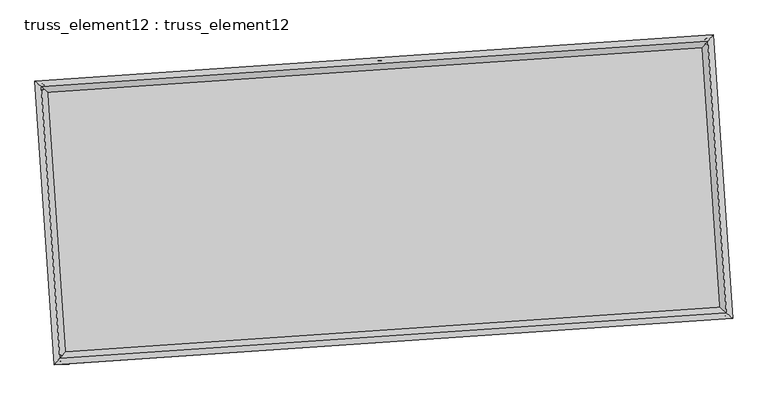
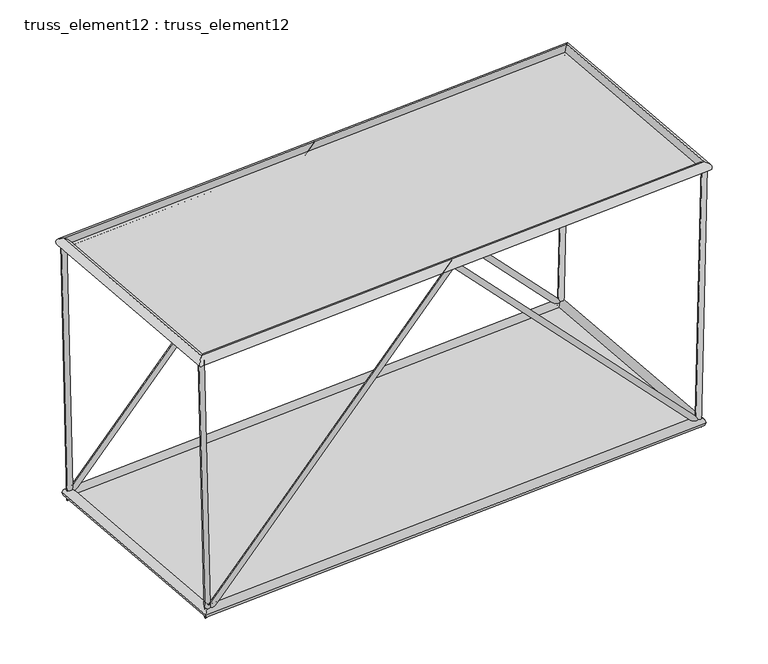
"""IFC4 building model written with IfcOpenShell, lengths in millimetres: plate geometry, truss_element12 : truss_element12."""

from ifc_helpers import new_model, si_unit, frame, origin, origin_with_axes, place, context, project, spatial, polyline, circle_curve, ellipse_curve, outline, extrude, source, transform, mapped, element, save
from ifc_brep_helpers import plane_surface, cylinder_surface, advanced_brep


def truss_element12_truss_element12_fedef946(model_context):
    return source(origin(), model_context, "Body", "SolidModel", [
        advanced_brep(
        [(-3782.029021, 2268.2402197, 4999.7937205), (-3881.1049687, 2254.8808593, 4997.4519118), (-3667.7673536, 2276.0312884, 121.2284017), (-3761.2195292, 2263.0553917, -121.2284017), (1063.6545258, 2598.6489605, 5070.7379406), (1064.1036954, 2592.0758396, 4926.5107213), (5795.2031248, 2921.2752732, 121.229281), (5889.5578522, 2921.1052153, -121.229281), (5909.3390115, 2929.0577654, 4999.7954616), (6009.3114208, 2929.2707559, 4997.4562298)],
        [
            (0, 1, circle_curve(frame((-3831.5669949, 2261.5605395, 4998.6228161), z_axis=(-0.02341471068854239, -0.0015965601142035673, 0.9997245632268789), x_axis=(-0.1335941952691201, 0.9910349136664861, -0.0015462485106522157)), 50.0)),
            (1, 0, circle_curve(frame((-3831.5669949, 2261.5605395, 4998.6228161), z_axis=(-0.02341471068854239, -0.0015965601142035673, 0.9997245632268789), x_axis=(-0.1335941952691201, 0.9910349136664861, -0.0015462485106522157)), 50.0)),
            (0, 2),
            (2, 3, ellipse_curve(frame((-3714.4934414, 2269.54334, 0.0), z_axis=(-0.9300661480063914, -0.06341767512013644, 0.36187727037617307), x_axis=(0.3610389440712066, 0.024617873158703073, 0.9322257458282786)), 130.3250571, 50.0)),
            (3, 1),
            (3, 2, ellipse_curve(frame((-3714.4934414, 2269.54334, 0.0), z_axis=(-0.9300661480063914, -0.06341767512013644, 0.36187727037617307), x_axis=(0.3610389440712066, 0.024617873158703073, 0.9322257458282786)), 130.3250571, 50.0)),
            (2, 4),
            (4, 5, ellipse_curve(frame((1063.8791106, 2595.3624001, 4998.6243309), z_axis=(-0.9976833960522568, -0.06802823822716046, -6.7338070324165216e-06), x_axis=(6.718207468311702e-06, 4.5808902877525703e-07, -0.9999999999773279)), 72.2706352, 50.0)),
            (5, 3),
            (5, 4, ellipse_curve(frame((1063.8791106, 2595.3624001, 4998.6243309), z_axis=(-0.9976833960522568, -0.06802823822716046, -6.7338070324165216e-06), x_axis=(6.718207468311702e-06, 4.5808902877525703e-07, -0.9999999999773279)), 72.2706352, 50.0)),
            (4, 6),
            (6, 7, ellipse_curve(frame((5842.3804885, 2921.1902443, 0.0), z_axis=(-0.9300590534640555, -0.06341719137026322, -0.3618955884067292), x_axis=(-0.36105721966614135, -0.02461911930204943, 0.9322186348125355)), 130.3269965, 50.0)),
            (7, 5),
            (7, 6, ellipse_curve(frame((5842.3804885, 2921.1902443, 0.0), z_axis=(-0.9300590534640555, -0.06341719137026322, -0.3618955884067292), x_axis=(-0.36105721966614135, -0.02461911930204943, 0.9322186348125355)), 130.3269965, 50.0)),
            (8, 9, circle_curve(frame((5959.3252161, 2929.1642607, 4998.6258457), z_axis=(0.023388945526827118, 0.0015948032857688488, 0.9997251691488132), x_axis=(-0.002166625472093405, 0.9999964600479803, -0.0015445470442767841)), 50.0)),
            (9, 8, circle_curve(frame((5959.3252161, 2929.1642607, 4998.6258457), z_axis=(0.023388945526827118, 0.0015948032857688488, 0.9997251691488132), x_axis=(-0.002166625472093405, 0.9999964600479803, -0.0015445470442767841)), 50.0)),
            (6, 8),
            (9, 7),
        ],
        [
            plane_surface(frame((-3831.5669949, 2311.5604757, 4998.702666), z_axis=(-0.023414710688541198, -0.0015965601141989434, 0.999724563226879), x_axis=(0.9997258380793066, -3.739324497509243e-05, 0.02341468083005437))),
            cylinder_surface(frame((-3831.5669949, 2261.5605395, 4998.6228161), z_axis=(-0.02341471068854239, -0.0015965601142035673, 0.9997245632268789), x_axis=(-0.1335941952691201, 0.9910349136664861, -0.0015462485106522157)), 50.0),
            cylinder_surface(frame((-3714.4934414, 2269.54334, 0.0), z_axis=(-0.6902363467958819, -0.047064592654016545, -0.7220517361520478), x_axis=(-0.020418619460760453, 0.9987519259602177, -0.04558146959096984)), 50.0),
            cylinder_surface(frame((1063.8791106, 2595.3624001, 4998.6243309), z_axis=(-0.6902460485200185, -0.04706525417770545, 0.722042418665059), x_axis=(-0.11534162865299183, 0.9922794867995385, -0.04558211026839251)), 50.0),
            plane_surface(frame((5959.3252161, 2879.1643243, 4998.7056077), z_axis=(0.023388945526829154, 0.0015948032857737223, 0.9997251691488129), x_axis=(0.999726441196362, -3.731097392289939e-05, -0.023388915766837215))),
            cylinder_surface(frame((5842.3804885, 2921.1902443, 0.0), z_axis=(-0.023388945526827118, -0.0015948032857688488, -0.9997251691488132), x_axis=(-0.002166625472093405, 0.9999964600479803, -0.0015445470442767841)), 50.0),
        ],
        [
            (0, [[1, 2]]),
            (1, [[-1, 3, 4, 5]]),
            (1, [[-2, -5, 6, -3]]),
            (2, [[-4, 7, 8, 9]]),
            (2, [[-6, -9, 10, -7]]),
            (3, [[-8, 11, 12, 13]]),
            (3, [[-10, -13, 14, -11]]),
            (4, [[15, 16]]),
            (5, [[-12, 17, -16, 18]]),
            (5, [[-14, -18, -15, -17]]),
        ],
    ),
        advanced_brep(
        [(-3509.9160681, -1722.4933646, 4999.7937205), (-3608.9920158, -1735.852725, 4997.4519118), (-3395.6544007, -1714.7022959, 121.2284017), (-3489.1065763, -1727.6781926, -121.2284017), (1335.7674788, -1392.0846238, 5070.7379406), (1336.2166483, -1398.6577447, 4926.5107213), (6067.3160777, -1069.4583111, 121.229281), (6161.6708052, -1069.628369, -121.229281), (6181.4519644, -1061.6758189, 4999.7954616), (6281.4243737, -1061.4628284, 4997.4562298)],
        [
            (0, 1, circle_curve(frame((-3559.4540419, -1729.1730448, 4998.6228161), z_axis=(-0.023414710688542402, -0.0015965601142035601, 0.999724563226879), x_axis=(-0.13359419526911945, 0.9910349136664863, -0.001546248510652208)), 50.0)),
            (1, 0, circle_curve(frame((-3559.4540419, -1729.1730448, 4998.6228161), z_axis=(-0.023414710688542402, -0.0015965601142035601, 0.999724563226879), x_axis=(-0.13359419526911945, 0.9910349136664863, -0.001546248510652208)), 50.0)),
            (0, 2),
            (2, 3, ellipse_curve(frame((-3442.3804885, -1721.1902443, 0.0), z_axis=(-0.9300661480063912, -0.06341767512013613, 0.36187727037617334), x_axis=(0.3610389440712068, 0.024617873158702973, 0.9322257458282784)), 130.3250571, 50.0)),
            (3, 1),
            (3, 2, ellipse_curve(frame((-3442.3804885, -1721.1902443, 0.0), z_axis=(-0.9300661480063912, -0.06341767512013613, 0.36187727037617334), x_axis=(0.3610389440712068, 0.024617873158702973, 0.9322257458282784)), 130.3250571, 50.0)),
            (2, 4),
            (4, 5, ellipse_curve(frame((1335.9920636, -1395.3711842, 4998.6243309), z_axis=(-0.997683396052257, -0.0680282382271604, -6.733807032095577e-06), x_axis=(6.718207468465462e-06, 4.5808902903472784e-07, -0.9999999999773279)), 72.2706352, 50.0)),
            (5, 3),
            (5, 4, ellipse_curve(frame((1335.9920636, -1395.3711842, 4998.6243309), z_axis=(-0.997683396052257, -0.0680282382271604, -6.733807032095577e-06), x_axis=(6.718207468465462e-06, 4.5808902903472784e-07, -0.9999999999773279)), 72.2706352, 50.0)),
            (4, 6),
            (6, 7, ellipse_curve(frame((6114.4934414, -1069.54334, 0.0), z_axis=(-0.9300590534640557, -0.06341719137026328, -0.3618955884067287), x_axis=(-0.36105721966614074, -0.02461911930204951, 0.9322186348125356)), 130.3269965, 50.0)),
            (7, 5),
            (7, 6, ellipse_curve(frame((6114.4934414, -1069.54334, 0.0), z_axis=(-0.9300590534640557, -0.06341719137026328, -0.3618955884067287), x_axis=(-0.36105721966614074, -0.02461911930204951, 0.9322186348125356)), 130.3269965, 50.0)),
            (8, 9, circle_curve(frame((6231.4381691, -1061.5693236, 4998.6258457), z_axis=(0.023388945526827663, 0.0015948032857688026, 0.999725169148813), x_axis=(-0.002166625472094084, 0.9999964600479802, -0.001544547044276721)), 50.0)),
            (9, 8, circle_curve(frame((6231.4381691, -1061.5693236, 4998.6258457), z_axis=(0.023388945526827663, 0.0015948032857688026, 0.999725169148813), x_axis=(-0.002166625472094084, 0.9999964600479802, -0.001544547044276721)), 50.0)),
            (6, 8),
            (9, 7),
        ],
        [
            plane_surface(frame((-3559.4540419, -1679.1731086, 4998.702666), z_axis=(-0.023414710688541198, -0.0015965601141989477, 0.999724563226879), x_axis=(0.9997258380793066, -3.739324497509243e-05, 0.02341468083005437))),
            cylinder_surface(frame((-3559.4540419, -1729.1730448, 4998.6228161), z_axis=(-0.023414710688542402, -0.0015965601142035601, 0.999724563226879), x_axis=(-0.13359419526911945, 0.9910349136664863, -0.001546248510652208)), 50.0),
            cylinder_surface(frame((-3442.3804885, -1721.1902443, 0.0), z_axis=(-0.6902363467958823, -0.047064592654016364, -0.7220517361520478), x_axis=(-0.020418619460760457, 0.9987519259602178, -0.04558146959096958)), 50.0),
            cylinder_surface(frame((1335.9920636, -1395.3711842, 4998.6243309), z_axis=(-0.6902460485200181, -0.04706525417770555, 0.7220424186650592), x_axis=(-0.11534162865299175, 0.9922794867995385, -0.04558211026839221)), 50.0),
            plane_surface(frame((6231.4381691, -1111.56926, 4998.7056077), z_axis=(0.02338894552682561, 0.0015948032857737312, 0.9997251691488132), x_axis=(0.9997264411963621, -3.731097392245531e-05, -0.023388915766833666))),
            cylinder_surface(frame((6114.4934414, -1069.54334, 0.0), z_axis=(-0.023388945526827663, -0.0015948032857688026, -0.999725169148813), x_axis=(-0.002166625472094084, 0.9999964600479802, -0.001544547044276721)), 50.0),
        ],
        [
            (0, [[1, 2]]),
            (1, [[-1, 3, 4, 5]]),
            (1, [[-2, -5, 6, -3]]),
            (2, [[-4, 7, 8, 9]]),
            (2, [[-6, -9, 10, -7]]),
            (3, [[-8, 11, 12, 13]]),
            (3, [[-10, -13, 14, -11]]),
            (4, [[15, 16]]),
            (5, [[-12, 17, -16, 18]]),
            (5, [[-14, -18, -15, -17]]),
        ],
    ),
        advanced_brep(
        [(-3559.4532557, -1729.1721734, 4908.6228161), (-3559.4548282, -1729.1739162, 5088.6228161), (-3831.5678921, 2261.5612961, 5088.6228161), (-3831.5660976, 2261.5597829, 4908.6228161), (5959.3259469, 2929.1651283, 5088.6258457), (5959.3244853, 2929.1633931, 4908.6258457), (6231.4390108, -1061.570084, 5088.6258457), (6231.4373273, -1061.5685632, 4908.6258457)],
        [
            (0, 1, ellipse_curve(frame((-3559.4540419, -1729.1730448, 4998.6228161), z_axis=(-0.7535719234054217, 0.657365466278086, -2.182941780963091e-07), x_axis=(-0.65736546627805, -0.7535719234054532, -2.1829417809634472e-07)), 127.2792206, 90.0)),
            (1, 2),
            (2, 3, ellipse_curve(frame((-3831.5669949, 2261.5605395, 4998.6228161), z_axis=(-0.65736546627805, -0.7535719234054532, -2.1829417809637778e-07), x_axis=(0.7535719234054218, -0.6573654662780859, 2.1829417809634224e-07)), 127.2792206, 90.0)),
            (3, 0),
            (1, 0, ellipse_curve(frame((-3559.4540419, -1729.1730448, 4998.6228161), z_axis=(-0.7535719234054217, 0.657365466278086, -2.182941780963091e-07), x_axis=(-0.65736546627805, -0.7535719234054532, -2.1829417809634472e-07)), 127.2792206, 90.0)),
            (3, 2, ellipse_curve(frame((-3831.5669949, 2261.5605395, 4998.6228161), z_axis=(-0.65736546627805, -0.7535719234054532, -2.1829417809637778e-07), x_axis=(0.7535719234054218, -0.6573654662780859, 2.1829417809634224e-07)), 127.2792206, 90.0)),
            (2, 4),
            (4, 5, ellipse_curve(frame((5959.3252161, 2929.1642607, 4998.6258457), z_axis=(-0.7535719234054216, 0.6573654662780861, -2.1829417809637545e-07), x_axis=(-0.6573654662780505, -0.7535719234054526, -2.182941780963446e-07)), 127.2792206, 90.0)),
            (5, 3),
            (5, 4, ellipse_curve(frame((5959.3252161, 2929.1642607, 4998.6258457), z_axis=(-0.7535719234054216, 0.6573654662780861, -2.1829417809637545e-07), x_axis=(-0.6573654662780505, -0.7535719234054526, -2.182941780963446e-07)), 127.2792206, 90.0)),
            (4, 6),
            (6, 7, ellipse_curve(frame((6231.4381691, -1061.5693236, 4998.6258457), z_axis=(0.6573654662780504, 0.7535719234054529, 2.1829417809631145e-07), x_axis=(-0.7535719234054216, 0.6573654662780863, -2.1829417809634234e-07)), 127.2792206, 90.0)),
            (7, 5),
            (7, 6, ellipse_curve(frame((6231.4381691, -1061.5693236, 4998.6258457), z_axis=(0.6573654662780504, 0.7535719234054529, 2.1829417809631145e-07), x_axis=(-0.7535719234054216, 0.6573654662780863, -2.1829417809634234e-07)), 127.2792206, 90.0)),
            (6, 1),
            (0, 7),
        ],
        [
            cylinder_surface(frame((-3559.4540419, -1729.1730448, 4998.6228161), z_axis=(0.06802823822869762, -0.997683396074877, 0.0), x_axis=(-0.9976833960310402, -0.06802823822570855, -9.37427355396142e-06)), 90.0),
            cylinder_surface(frame((-3831.5669949, 2261.5605395, 4998.6228161), z_axis=(-0.9976833960748294, -0.06802823822869407, -3.0871458725096017e-07), x_axis=(-0.06802823822310969, 0.9976833960340703, -9.06555896672317e-06)), 90.0),
            cylinder_surface(frame((5959.3252161, 2929.1642607, 4998.6258457), z_axis=(-0.06802823822869693, 0.9976833960748771, 0.0), x_axis=(0.9976833960366246, 0.06802823822608864, -8.75684437948492e-06)), 90.0),
            cylinder_surface(frame((6231.4381691, -1061.5693236, 4998.6258457), z_axis=(0.9976833960748294, 0.06802823822869393, 3.0871458725091337e-07), x_axis=(0.06802823822869393, -0.9976833960336895, -9.065558966723174e-06)), 90.0),
        ],
        [
            (0, [[1, 2, 3, 4]]),
            (0, [[5, -4, 6, -2]]),
            (1, [[-3, 7, 8, 9]]),
            (1, [[-6, -9, 10, -7]]),
            (2, [[-8, 11, 12, 13]]),
            (2, [[-10, -13, 14, -11]]),
            (3, [[-12, 15, -1, 16]]),
            (3, [[-14, -16, -5, -15]]),
        ],
    ),
        advanced_brep(
        [(-3358.7115243, -1625.2761972, 0.0), (-3526.0494527, -1817.1042913, 0.0), (-3810.4074885, 2353.2123043, 0.0), (-3618.5793943, 2185.8743758, 0.0), (5926.0494527, 3017.1042913, 0.0), (5758.7115243, 2825.2761972, 0.0), (6210.4074885, -1153.2123043, 0.0), (6018.5793943, -985.8743758, 0.0)],
        [
            (0, 1, ellipse_curve(frame((-3442.3804885, -1721.1902443, 0.0), z_axis=(-0.753571923405459, 0.6573654662780796, 0.0), x_axis=(-0.6573654662780796, -0.7535719234054591, 0.0)), 127.2792206, 90.0)),
            (1, 2),
            (2, 3, ellipse_curve(frame((-3714.4934414, 2269.54334, 0.0), z_axis=(-0.6573654662780795, -0.753571923405459, 0.0), x_axis=(0.7535719234054589, -0.6573654662780798, 0.0)), 127.2792206, 90.0)),
            (3, 0),
            (1, 0, ellipse_curve(frame((-3442.3804885, -1721.1902443, 0.0), z_axis=(-0.753571923405459, 0.6573654662780796, 0.0), x_axis=(-0.6573654662780796, -0.7535719234054591, 0.0)), 127.2792206, 90.0)),
            (3, 2, ellipse_curve(frame((-3714.4934414, 2269.54334, 0.0), z_axis=(-0.6573654662780795, -0.753571923405459, 0.0), x_axis=(0.7535719234054589, -0.6573654662780798, 0.0)), 127.2792206, 90.0)),
            (2, 4),
            (4, 5, ellipse_curve(frame((5842.3804885, 2921.1902443, 0.0), z_axis=(-0.753571923405459, 0.6573654662780796, 0.0), x_axis=(-0.6573654662780795, -0.753571923405459, 0.0)), 127.2792206, 90.0)),
            (5, 3),
            (5, 4, ellipse_curve(frame((5842.3804885, 2921.1902443, 0.0), z_axis=(-0.753571923405459, 0.6573654662780796, 0.0), x_axis=(-0.6573654662780795, -0.753571923405459, 0.0)), 127.2792206, 90.0)),
            (4, 6),
            (6, 7, ellipse_curve(frame((6114.4934414, -1069.54334, 0.0), z_axis=(0.6573654662780796, 0.7535719234054591, 0.0), x_axis=(-0.753571923405459, 0.6573654662780795, 0.0)), 127.2792206, 90.0)),
            (7, 5),
            (7, 6, ellipse_curve(frame((6114.4934414, -1069.54334, 0.0), z_axis=(0.6573654662780796, 0.7535719234054591, 0.0), x_axis=(-0.753571923405459, 0.6573654662780795, 0.0)), 127.2792206, 90.0)),
            (6, 1),
            (0, 7),
        ],
        [
            cylinder_surface(frame((-3442.3804885, -1721.1902443, 0.0), z_axis=(0.0680282382287029, -0.9976833960748764, 0.0), x_axis=(-0.9976833960748764, -0.0680282382287029, 0.0)), 90.0),
            cylinder_surface(frame((-3714.4934414, 2269.54334, 0.0), z_axis=(-0.9976833960748764, -0.06802823822870277, 0.0), x_axis=(-0.06802823822870277, 0.9976833960748764, 0.0)), 90.0),
            cylinder_surface(frame((5842.3804885, 2921.1902443, 0.0), z_axis=(-0.06802823822870296, 0.9976833960748764, 0.0), x_axis=(0.9976833960748764, 0.06802823822870296, 0.0)), 90.0),
            cylinder_surface(frame((6114.4934414, -1069.54334, 0.0), z_axis=(0.9976833960748764, 0.06802823822870276, 0.0), x_axis=(0.06802823822870276, -0.9976833960748764, 0.0)), 90.0),
        ],
        [
            (0, [[1, 2, 3, 4]]),
            (0, [[5, -4, 6, -2]]),
            (1, [[-3, 7, 8, 9]]),
            (1, [[-6, -9, 10, -7]]),
            (2, [[-8, 11, 12, 13]]),
            (2, [[-10, -13, 14, -11]]),
            (3, [[-12, 15, -1, 16]]),
            (3, [[-14, -16, -5, -15]]),
        ],
    ),
        extrude(outline(polyline([(-3442.3804885, -1721.1902443), (-3714.4934414, 2269.54334), (5842.3804885, 2921.1902443), (6114.4934414, -1069.54334), (-3442.3804885, -1721.1902443)])), origin_with_axes(), (0.0, 0.0, 1.0), 20.0),
        extrude(outline(polyline([(-2000.0, 4906.8132483), (2000.0000001, 4906.8132484), (2000.0000001, -4906.8132483), (-2000.0, -4906.8132484), (-2000.0, 4906.8132483)])), frame((1199.9355871, 599.9956079, 4998.6243309), z_axis=(-3.0799941782636826e-07, -2.100130948618238e-08, 0.9999999999999524), x_axis=(-0.06802823822870281, 0.9976833960748764, 0.0)), (0.0, 0.0, 1.0), 20.0),
    ])


if __name__ == "__main__":
    model = new_model("IFC4")
    model_context = context("Model", 3, world=origin())
    ifc_project = project(units=[si_unit("LENGTHUNIT", "METRE", prefix="MILLI")], contexts=[model_context])
    site = spatial("IfcSite", under=ifc_project)
    building = spatial("IfcBuilding", under=site)
    placement = place(None, origin())
    truss_element12_truss_element12_shape = truss_element12_truss_element12_fedef946(model_context)
    element("IfcPlate", 1, ObjectType="truss_element12 : truss_element12", at=placement, inside=building, context=model_context, shape_type="MappedRepresentation", body=[
        mapped(truss_element12_truss_element12_shape, transform((0.0, 0.0, 0.0), x_axis=(1.0, 0.0, 0.0), y_axis=(0.0, 1.0, 0.0), z_axis=(0.0, 0.0, 1.0))),
    ])
    save(model, "model.ifc")

# Revit data of these elements
# Type "truss_element12 : truss_element12"
#   steellbar1 = 90 mm
#   steelbar2 = 50 mm
#   offset1 = 5000 mm
#   M = Default Roof
# Element 1 (IfcPlate, "truss_element12 : truss_element12")
#   Materials on its faces: "Default Roof"
# Materials
#   "Default Roof": class "Miscellaneous", colour RGB 0 127 0, transparency 0, Comments = "Rendering appearance not upgraded Rendering appearance not upgraded ", Cost = 0
